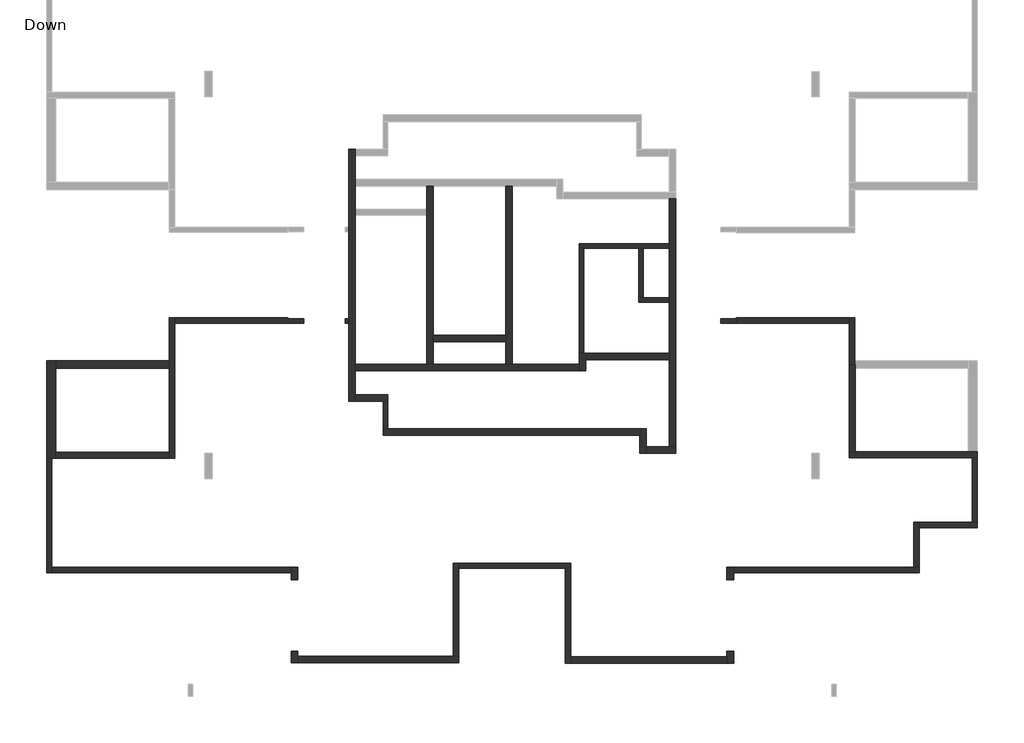
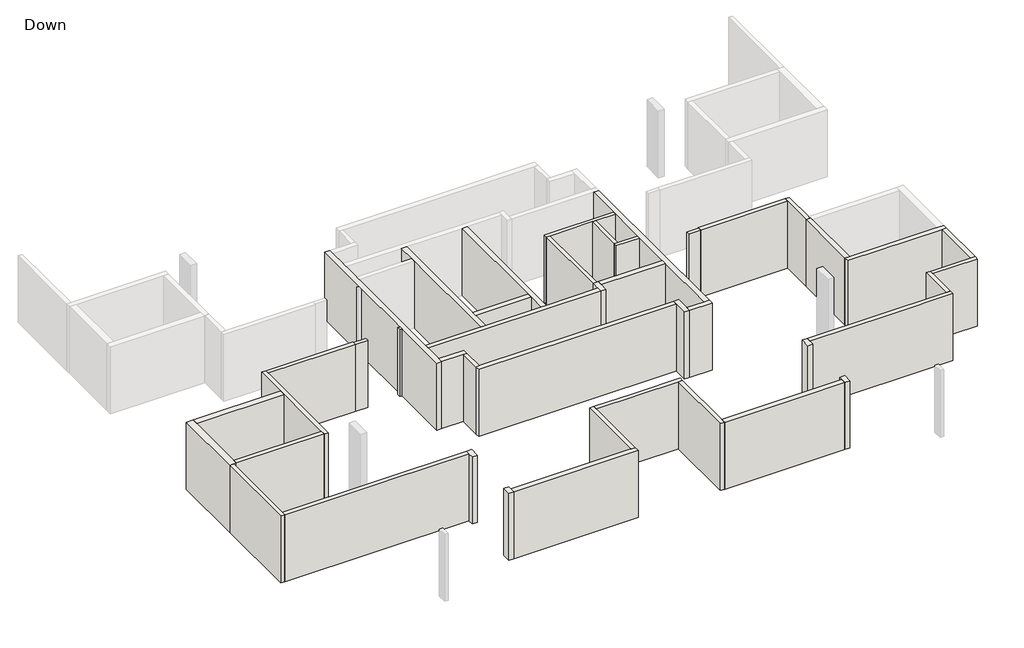
# One storey, part 1 of 2: 44 walls.
# Revit data of these elements (continued)
# Element 38 (IfcWall, "22") (continued)
#   Comments = ""
#   Mark = "W63"
#   SOFiSTiK_EdgeZones = "W63"
#   SOFiSTiK_AMG_Comments = ""
#   Top Offset = 0 cm
#   Base Offset = 0 cm
#   wall height = 307 cm
#   SOFiSTiK_AMG_Scheduled = yes
#   SOFiSTiK_AMG_Adjusted = yes
#   Phase Created = New Construction
#   Base Constraint = Down
#   Top Constraint = Typical Floor
#   Materials on its faces: "Concrete"
# Element 39 (IfcWall, "22")
#   Comments = ""
#   Mark = "W68"
#   SOFiSTiK_EdgeZones = "W68"
#   SOFiSTiK_AMG_Comments = ""
#   Top Offset = 0 cm
#   Base Offset = 0 cm
#   wall height = 307 cm
#   SOFiSTiK_AMG_Scheduled = yes
#   SOFiSTiK_AMG_Adjusted = yes
#   Phase Created = New Construction
#   Base Constraint = Down
#   Top Constraint = Typical Floor
#   Materials on its faces: "Concrete"
# Element 40 (IfcWall, "22")
#   Comments = ""
#   Mark = "W69"
#   SOFiSTiK_EdgeZones = "W69"
#   SOFiSTiK_AMG_Comments = ""
#   Top Offset = 0 cm
#   Base Offset = 0 cm
#   wall height = 307 cm
#   SOFiSTiK_AMG_Scheduled = yes
#   SOFiSTiK_AMG_Adjusted = yes
#   Phase Created = New Construction
#   Base Constraint = Down
#   Top Constraint = Typical Floor
#   Materials on its faces: "Concrete"
# Element 41 (IfcWall, "22")
#   Comments = ""
#   Mark = "W70"
#   SOFiSTiK_EdgeZones = "W70"
#   SOFiSTiK_AMG_Comments = ""
#   Top Offset = 0 cm
#   Base Offset = 0 cm
#   wall height = 307 cm
#   SOFiSTiK_AMG_Scheduled = yes
#   SOFiSTiK_AMG_Adjusted = yes
#   Phase Created = New Construction
#   Base Constraint = Down
#   Top Constraint = Typical Floor
#   Materials on its faces: "Concrete"
# Element 42 (IfcWall, "22")
#   Comments = ""
#   Mark = "W71"
#   SOFiSTiK_EdgeZones = "W71"
#   SOFiSTiK_AMG_Comments = ""
#   Top Offset = 0 cm
#   Base Offset = 0 cm
#   wall height = 307 cm
#   SOFiSTiK_AMG_Scheduled = yes
#   SOFiSTiK_AMG_Adjusted = yes
#   Phase Created = New Construction
#   Base Constraint = Down
#   Top Constraint = Typical Floor
#   Materials on its faces: "Concrete"
# Element 43 (IfcWall, "25")
#   Comments = ""
#   Mark = "W29"
#   SOFiSTiK_EdgeZones = "W29"
#   SOFiSTiK_AMG_Comments = ""
#   Top Offset = 0 cm
#   Base Offset = 0 cm
#   wall height = 307 cm
#   SOFiSTiK_AMG_Scheduled = yes
#   SOFiSTiK_AMG_Adjusted = yes
#   Phase Created = New Construction
#   Base Constraint = Down
#   Top Constraint = Typical Floor
#   Materials on its faces: "Concrete"
# Element 44 (IfcWall, "30")
#   Comments = ""
#   Mark = "W1"
#   SOFiSTiK_EdgeZones = "W1"
#   SOFiSTiK_AMG_Comments = ""
#   Top Offset = 0 cm
#   Base Offset = 0 cm
#   wall height = 307 cm
#   SOFiSTiK_AMG_Scheduled = yes
#   SOFiSTiK_AMG_Adjusted = yes
#   Phase Created = New Construction
#   Base Constraint = Down
#   Top Constraint = Typical Floor
#   Materials on its faces: "Concrete"
# Materials
#   "Concrete": class "Concrete", colour RGB 192 192 192, transparency 0, Keynote = "01000", Description = "Cast-in-place concrete", Cost = 0
